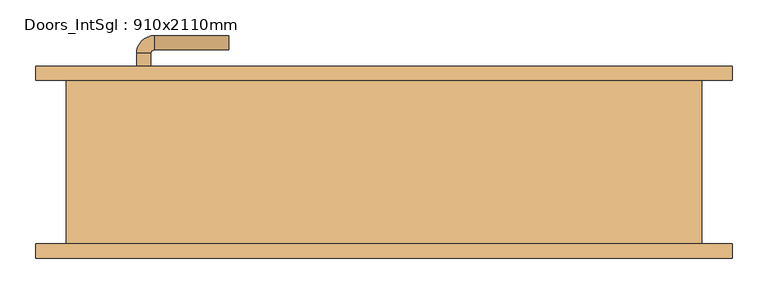
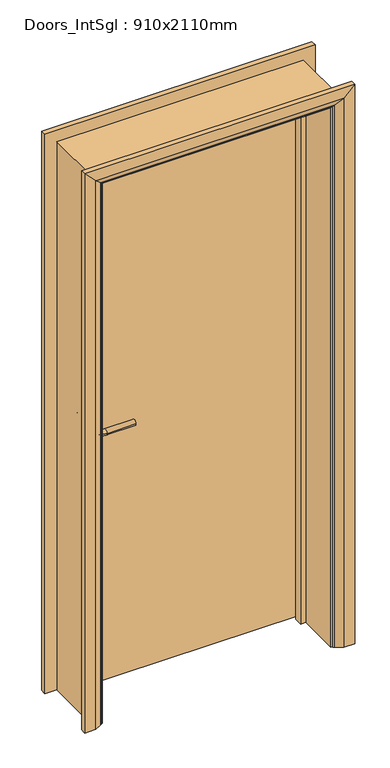
"""IFC4 building model written with IfcOpenShell, lengths in millimetres: door geometry, Doors_IntSgl : 910x2110mm."""

from ifc_helpers import new_model, si_unit, point, frame, frame_2d, origin, place, context, project, spatial, polyline, circle_curve, ellipse_curve, trimmed, segment, composite_curve, outline, extrude, faceted_brep, source, transform, mapped, element, save
from ifc_brep_helpers import plane_surface, cylinder_surface, revolved_surface, advanced_brep


def doors_intsgl_910x2110mm_0ed93a32(model_context):
    return source(origin(), model_context, "Body", "SolidModel", [
        advanced_brep(
        [(-348.0, 69.0, 1000.0), (-328.0, 69.0, 1000.0), (-328.0, 39.0, 1000.0), (-348.0, 39.0, 1000.0), (-323.0, 34.0, 1000.0), (-323.0, 14.0, 1000.0), (-218.0, 14.0, 1000.0), (-218.0, 34.0, 1000.0)],
        [
            (0, 1, circle_curve(frame((-338.0, 69.0, 1000.0), z_axis=(0.0, 1.0, 0.0), x_axis=(1.0, 0.0, 0.0)), 10.0)),
            (1, 0, circle_curve(frame((-338.0, 69.0, 1000.0), z_axis=(0.0, 1.0, 0.0), x_axis=(1.0, 0.0, 0.0)), 10.0)),
            (1, 2),
            (2, 3, circle_curve(frame((-338.0, 39.0, 1000.0), z_axis=(0.0, 1.0, 0.0), x_axis=(1.0, 0.0, 0.0)), 10.0)),
            (3, 0),
            (3, 2, circle_curve(frame((-338.0, 39.0, 1000.0), z_axis=(0.0, 1.0, 0.0), x_axis=(1.0, 0.0, 0.0)), 10.0)),
            (4, 5, circle_curve(frame((-323.0, 24.0, 1000.0), z_axis=(-1.0, 0.0, 0.0), x_axis=(0.0, 1.0, 0.0)), 10.0)),
            (5, 3, circle_curve(frame((-323.0, 39.0, 1000.0), z_axis=(0.0, 0.0, -1.0), x_axis=(-1.0, 0.0, 0.0)), 25.0)),
            (2, 4, circle_curve(frame((-323.0, 39.0, 1000.0), z_axis=(0.0, 0.0, 1.0), x_axis=(-1.0, 0.0, 0.0)), 5.0)),
            (5, 4, circle_curve(frame((-323.0, 24.0, 1000.0), z_axis=(-1.0, 0.0, 0.0), x_axis=(0.0, 1.0, 0.0)), 10.0)),
            (6, 7, circle_curve(frame((-218.0, 24.0, 1000.0), z_axis=(1.0, 0.0, 0.0), x_axis=(0.0, 1.0, 0.0)), 10.0)),
            (7, 6, circle_curve(frame((-218.0, 24.0, 1000.0), z_axis=(1.0, 0.0, 0.0), x_axis=(0.0, 1.0, 0.0)), 10.0)),
            (4, 7),
            (6, 5),
        ],
        [
            plane_surface(frame((-338.0, 69.0, 1000.0), z_axis=(0.0, 1.0, 0.0), x_axis=(0.0, 0.0, 1.0))),
            cylinder_surface(frame((-338.0, 69.0, 1000.0), z_axis=(0.0, 1.0, 0.0), x_axis=(1.0, 0.0, 0.0)), 10.0),
            revolved_surface(trimmed(ellipse_curve(frame((-338.0, 39.0, 1000.0), z_axis=(0.0, -1.0, 0.0), x_axis=(1.0, 0.0, 0.0)), 10.0, 10.0), [point((-348.0, 39.0, 1000.0))], [point((-328.0, 39.0, 1000.0))], True, "CARTESIAN"), (-323.0, 39.0, 1000.0), (0.0, 0.0, -1.0)),
            revolved_surface(trimmed(ellipse_curve(frame((-338.0, 39.0, 1000.0), z_axis=(0.0, -1.0, 0.0), x_axis=(1.0, 0.0, 0.0)), 10.0, 10.0), [point((-328.0, 39.0, 1000.0))], [point((-348.0, 39.0, 1000.0))], True, "CARTESIAN"), (-323.0, 39.0, 1000.0), (0.0, 0.0, -1.0)),
            plane_surface(frame((-218.0, 24.0, 1000.0), z_axis=(1.0, 0.0, 0.0), x_axis=(0.0, 0.0, 1.0))),
            cylinder_surface(frame((-323.0, 24.0, 1000.0), z_axis=(-1.0, 0.0, 0.0), x_axis=(0.0, 1.0, 0.0)), 10.0),
        ],
        [
            (0, [[1, 2]]),
            (1, [[3, 4, 5, -2]]),
            (1, [[-5, 6, -3, -1]]),
            (2, [[7, 8, -4, 9]]),
            (3, [[10, -9, -6, -8]]),
            (4, [[11, 12]]),
            (5, [[13, -11, 14, -7]]),
            (5, [[-14, -12, -13, -10]]),
        ],
    ),
        extrude(outline(composite_curve([segment(trimmed(circle_curve(frame_2d((1000.0, -340.5)), 30.0), [point((1000.0, -370.5))], [point((1000.0, -310.5))], False, "CARTESIAN"), True, "CONTINUOUS"), segment(trimmed(circle_curve(frame_2d((1000.0, -340.5)), 30.0), [point((1000.0, -310.5))], [point((1000.0, -370.5))], False, "CARTESIAN"), True, "CONTINUOUS")], self_intersect=False)), frame((0.0, 69.0, 0.0), z_axis=(0.0, 1.0, 0.0), x_axis=(0.0, 0.0, 1.0)), (0.0, 0.0, 1.0), 8.0),
        advanced_brep(
        [(-348.0, 123.0, 1000.0), (-328.0, 123.0, 1000.0), (-348.0, 153.0, 1000.0), (-328.0, 153.0, 1000.0), (-323.0, 158.0, 1000.0), (-323.0, 178.0, 1000.0), (-218.0, 178.0, 1000.0), (-218.0, 158.0, 1000.0)],
        [
            (0, 1, circle_curve(frame((-338.0, 123.0, 1000.0), z_axis=(0.0, -1.0, 0.0), x_axis=(1.0, 0.0, 0.0)), 10.0)),
            (1, 0, circle_curve(frame((-338.0, 123.0, 1000.0), z_axis=(0.0, -1.0, 0.0), x_axis=(1.0, 0.0, 0.0)), 10.0)),
            (0, 2),
            (2, 3, circle_curve(frame((-338.0, 153.0, 1000.0), z_axis=(0.0, -1.0, 0.0), x_axis=(1.0, 0.0, 0.0)), 10.0)),
            (3, 1),
            (3, 2, circle_curve(frame((-338.0, 153.0, 1000.0), z_axis=(0.0, -1.0, 0.0), x_axis=(1.0, 0.0, 0.0)), 10.0)),
            (4, 3, circle_curve(frame((-323.0, 153.0, 1000.0), z_axis=(0.0, 0.0, 1.0), x_axis=(-1.0, 0.0, 0.0)), 5.0)),
            (2, 5, circle_curve(frame((-323.0, 153.0, 1000.0), z_axis=(0.0, 0.0, -1.0), x_axis=(-1.0, 0.0, 0.0)), 25.0)),
            (5, 4, circle_curve(frame((-323.0, 168.0, 1000.0), z_axis=(-1.0, 0.0, 0.0), x_axis=(0.0, -1.0, 0.0)), 10.0)),
            (4, 5, circle_curve(frame((-323.0, 168.0, 1000.0), z_axis=(-1.0, 0.0, 0.0), x_axis=(0.0, -1.0, 0.0)), 10.0)),
            (6, 7, circle_curve(frame((-218.0, 168.0, 1000.0), z_axis=(1.0, 0.0, 0.0), x_axis=(0.0, -1.0, 0.0)), 10.0)),
            (7, 6, circle_curve(frame((-218.0, 168.0, 1000.0), z_axis=(1.0, 0.0, 0.0), x_axis=(0.0, -1.0, 0.0)), 10.0)),
            (5, 6),
            (7, 4),
        ],
        [
            plane_surface(frame((-338.0, 123.0, 1000.0), z_axis=(0.0, -1.0, 0.0), x_axis=(0.0, 0.0, 1.0))),
            cylinder_surface(frame((-338.0, 123.0, 1000.0), z_axis=(0.0, -1.0, 0.0), x_axis=(1.0, 0.0, 0.0)), 10.0),
            revolved_surface(trimmed(ellipse_curve(frame((-338.0, 153.0, 1000.0), z_axis=(0.0, -1.0, 0.0), x_axis=(1.0, 0.0, 0.0)), 10.0, 10.0), [point((-348.0, 153.0, 1000.0))], [point((-328.0, 153.0, 1000.0))], True, "CARTESIAN"), (-323.0, 153.0, 1000.0), (0.0, 0.0, -1.0)),
            revolved_surface(trimmed(ellipse_curve(frame((-338.0, 153.0, 1000.0), z_axis=(0.0, -1.0, 0.0), x_axis=(1.0, 0.0, 0.0)), 10.0, 10.0), [point((-328.0, 153.0, 1000.0))], [point((-348.0, 153.0, 1000.0))], True, "CARTESIAN"), (-323.0, 153.0, 1000.0), (0.0, 0.0, -1.0)),
            plane_surface(frame((-218.0, 168.0, 1000.0), z_axis=(1.0, 0.0, 0.0), x_axis=(0.0, 0.0, 1.0))),
            cylinder_surface(frame((-323.0, 168.0, 1000.0), z_axis=(-1.0, 0.0, 0.0), x_axis=(0.0, -1.0, 0.0)), 10.0),
        ],
        [
            (0, [[1, 2]]),
            (1, [[-1, 3, 4, 5]]),
            (1, [[-2, -5, 6, -3]]),
            (2, [[7, -4, 8, 9]]),
            (3, [[-8, -6, -7, 10]]),
            (4, [[11, 12]]),
            (5, [[-9, 13, -12, 14]]),
            (5, [[-10, -14, -11, -13]]),
        ],
    ),
        extrude(outline(composite_curve([segment(trimmed(circle_curve(frame_2d((1000.0, -340.5)), 30.0), [point((1000.0, -370.5))], [point((1000.0, -310.5))], False, "CARTESIAN"), True, "CONTINUOUS"), segment(trimmed(circle_curve(frame_2d((1000.0, -340.5)), 30.0), [point((1000.0, -310.5))], [point((1000.0, -370.5))], False, "CARTESIAN"), True, "CONTINUOUS")], self_intersect=False)), frame((0.0, 115.0, 0.0), z_axis=(0.0, 1.0, 0.0), x_axis=(0.0, 0.0, 1.0)), (0.0, 0.0, 1.0), 8.0),
        extrude(outline(polyline([(413.0, 77.0), (-413.0, 77.0), (-413.0, 115.0), (413.0, 115.0), (413.0, 77.0)])), frame((0.0, 0.0, 8.0), z_axis=(0.0, 0.0, 1.0), x_axis=(1.0, 0.0, 0.0)), (0.0, 0.0, 1.0), 2060.0),
        advanced_brep(
        [(490.0, 135.0, 0.0), (490.0, 115.0, 0.0), (420.0, 115.0, 0.0), (424.0, 121.0, 0.0), (450.0, 135.0, 0.0), (490.0, 135.0, 2145.0), (490.0, 115.0, 2145.0), (-490.0, 115.0, 2145.0), (-490.0, 115.0, 0.0), (-420.0, 115.0, 0.0), (-420.0, 115.0, 2075.0), (420.0, 115.0, 2075.0), (424.0, 121.0, 2079.0), (450.0, 135.0, 2105.0), (-450.0, 135.0, 2105.0), (-450.0, 135.0, 0.0), (-490.0, 135.0, 0.0), (-490.0, 135.0, 2145.0), (-424.0, 121.0, 2079.0), (-424.0, 121.0, 0.0)],
        [
            (0, 1),
            (1, 2),
            (2, 3, circle_curve(frame((428.0, 114.0, 0.0), z_axis=(0.0, 0.0, -1.0), x_axis=(1.0, 0.0, 0.0)), 8.0622577)),
            (3, 4),
            (4, 0),
            (0, 5),
            (5, 6),
            (6, 1),
            (6, 7),
            (7, 8),
            (8, 9),
            (9, 10),
            (10, 11),
            (11, 2),
            (11, 12, ellipse_curve(frame((428.0, 114.0, 2083.0), z_axis=(0.7071067811865475, 0.0, -0.7071067811865475), x_axis=(-0.7071067811865474, 0.0, -0.7071067811865476)), 11.4017543, 8.0622577)),
            (12, 3),
            (12, 13),
            (13, 4),
            (13, 14),
            (14, 15),
            (15, 16),
            (16, 17),
            (17, 5),
            (17, 7),
            (10, 18, ellipse_curve(frame((-428.0, 114.0, 2083.0), z_axis=(0.7071067811865475, 0.0, 0.7071067811865475), x_axis=(0.7071067811865476, 0.0, -0.7071067811865474)), 11.4017543, 8.0622577)),
            (18, 12),
            (18, 14),
            (15, 19),
            (19, 9, circle_curve(frame((-428.0, 114.0, 0.0), z_axis=(0.0, 0.0, -1.0), x_axis=(-1.0, 0.0, 0.0)), 8.0622577)),
            (8, 16),
            (19, 18),
        ],
        [
            plane_surface(frame((420.0, 115.0, 0.0), z_axis=(0.0, 0.0, -1.0), x_axis=(0.0, -1.0, 0.0))),
            plane_surface(frame((490.0, 135.0, 0.0), z_axis=(1.0, 0.0, 0.0), x_axis=(0.0, 0.0, 1.0))),
            plane_surface(frame((490.0, 115.0, 0.0), z_axis=(0.0, -1.0, 0.0), x_axis=(0.0, 0.0, 1.0))),
            cylinder_surface(frame((428.0, 114.0, 0.0), z_axis=(0.0, 0.0, -1.0), x_axis=(1.0, 0.0, 0.0)), 8.0622577),
            plane_surface(frame((424.0, 121.0, 0.0), z_axis=(-0.4740998230350126, 0.880471099922178, 0.0), x_axis=(0.0, 0.0, 1.0))),
            plane_surface(frame((450.0, 135.0, 0.0), z_axis=(0.0, 1.0, 0.0), x_axis=(0.0, 0.0, 1.0))),
            plane_surface(frame((490.0, 135.0, 2145.0), z_axis=(0.0, 0.0, 1.0), x_axis=(-1.0, 0.0, 0.0))),
            cylinder_surface(frame((420.0, 114.0, 2083.0), z_axis=(1.0, 0.0, 0.0), x_axis=(0.0, 0.0, 1.0)), 8.0622577),
            plane_surface(frame((424.0, 121.0, 2079.0), z_axis=(0.0, 0.8804710999221764, -0.4740998230350154), x_axis=(-1.0, 0.0, 0.0))),
            plane_surface(frame((-420.0, 115.0, 0.0), z_axis=(0.0, 0.0, -1.0), x_axis=(0.0, -1.0, 0.0))),
            plane_surface(frame((-490.0, 135.0, 2145.0), z_axis=(-1.0, 0.0, 0.0), x_axis=(0.0, 0.0, -1.0))),
            cylinder_surface(frame((-428.0, 114.0, 2075.0), z_axis=(0.0, 0.0, 1.0), x_axis=(-1.0, 0.0, 0.0)), 8.0622577),
            plane_surface(frame((-424.0, 121.0, 2079.0), z_axis=(0.47409982303501824, 0.8804710999221749, 0.0), x_axis=(0.0, 0.0, -1.0))),
        ],
        [
            (0, [[1, 2, 3, 4, 5]]),
            (1, [[-1, 6, 7, 8]]),
            (2, [[-2, -8, 9, 10, 11, 12, 13, 14]]),
            (3, [[-3, -14, 15, 16]]),
            (4, [[-4, -16, 17, 18]]),
            (5, [[-5, -18, 19, 20, 21, 22, 23, -6]]),
            (6, [[-7, -23, 24, -9]]),
            (7, [[-15, -13, 25, 26]]),
            (8, [[-17, -26, 27, -19]]),
            (9, [[-21, 28, 29, -11, 30]]),
            (10, [[-24, -22, -30, -10]]),
            (11, [[-25, -12, -29, 31]]),
            (12, [[-27, -31, -28, -20]]),
        ],
    ),
        extrude(outline(polyline([(0.0, -415.0), (0.0, -396.0), (2051.0, -396.0), (2051.0, 396.0), (0.0, 396.0), (0.0, 415.0), (2070.0, 415.0), (2070.0, -415.0), (0.0, -415.0)])), frame((0.0, 43.0, 0.0), z_axis=(0.0, 1.0, 0.0), x_axis=(0.0, 0.0, 1.0)), (0.0, 0.0, 1.0), 32.0),
        advanced_brep(
        [(-490.0, -135.0, 0.0), (-490.0, -115.0, 0.0), (-420.0, -115.0, 0.0), (-424.0, -121.0, 0.0), (-450.0, -135.0, 0.0), (-490.0, -135.0, 2145.0), (-490.0, -115.0, 2145.0), (-420.0, -115.0, 2075.0), (-424.0, -121.0, 2079.0), (-450.0, -135.0, 2105.0), (490.0, -135.0, 2145.0), (490.0, -115.0, 2145.0), (420.0, -115.0, 2075.0), (424.0, -121.0, 2079.0), (450.0, -135.0, 2105.0), (490.0, -135.0, 0.0), (450.0, -135.0, 0.0), (424.0, -121.0, 0.0), (420.0, -115.0, 0.0), (490.0, -115.0, 0.0)],
        [
            (0, 1),
            (1, 2),
            (2, 3, circle_curve(frame((-428.0, -114.0, 0.0), z_axis=(0.0, 0.0, -1.0), x_axis=(-1.0, 0.0, 0.0)), 8.0622577)),
            (3, 4),
            (4, 0),
            (0, 5),
            (5, 6),
            (6, 1),
            (6, 7),
            (7, 2),
            (7, 8, ellipse_curve(frame((-428.0, -114.0, 2083.0), z_axis=(-0.7071067811865475, 0.0, -0.7071067811865475), x_axis=(0.7071067811865474, 0.0, -0.7071067811865476)), 11.4017543, 8.0622577)),
            (8, 3),
            (8, 9),
            (9, 4),
            (9, 5),
            (5, 10),
            (10, 11),
            (11, 6),
            (11, 12),
            (12, 7),
            (12, 13, ellipse_curve(frame((428.0, -114.0, 2083.0), z_axis=(-0.7071067811865475, 0.0, 0.7071067811865475), x_axis=(-0.7071067811865476, 0.0, -0.7071067811865474)), 11.4017543, 8.0622577)),
            (13, 8),
            (13, 14),
            (14, 9),
            (14, 10),
            (15, 16),
            (16, 17),
            (17, 18, circle_curve(frame((428.0, -114.0, 0.0), z_axis=(0.0, 0.0, -1.0), x_axis=(1.0, 0.0, 0.0)), 8.0622577)),
            (18, 19),
            (19, 15),
            (10, 15),
            (19, 11),
            (18, 12),
            (17, 13),
            (16, 14),
        ],
        [
            plane_surface(frame((-420.0, -187.8010989, 0.0), z_axis=(0.0, 0.0, -1.0), x_axis=(1.0, 0.0, 0.0))),
            plane_surface(frame((-490.0, -135.0, 0.0), z_axis=(-1.0, 0.0, 0.0), x_axis=(0.0, 0.0, 1.0))),
            plane_surface(frame((-490.0, -115.0, 0.0), z_axis=(0.0, 1.0, 0.0), x_axis=(0.0, 0.0, 1.0))),
            cylinder_surface(frame((-428.0, -114.0, 0.0), z_axis=(0.0, 0.0, -1.0), x_axis=(-1.0, 0.0, 0.0)), 8.0622577),
            plane_surface(frame((-424.0, -121.0, 0.0), z_axis=(0.4740998230350183, -0.8804710999221749, 0.0), x_axis=(0.0, 0.0, 1.0))),
            plane_surface(frame((-450.0, -135.0, 0.0), z_axis=(0.0, -1.0, 0.0), x_axis=(0.0, 0.0, 1.0))),
            plane_surface(frame((-490.0, -135.0, 2145.0), z_axis=(0.0, 0.0, 1.0), x_axis=(1.0, 0.0, 0.0))),
            plane_surface(frame((-490.0, -115.0, 2145.0), z_axis=(0.0, 1.0, 0.0), x_axis=(1.0, 0.0, 0.0))),
            cylinder_surface(frame((-420.0, -114.0, 2083.0), z_axis=(-1.0, 0.0, 0.0), x_axis=(0.0, 0.0, 1.0)), 8.0622577),
            plane_surface(frame((-424.0, -121.0, 2079.0), z_axis=(0.0, -0.8804710999221749, -0.4740998230350183), x_axis=(1.0, 0.0, 0.0))),
            plane_surface(frame((-450.0, -135.0, 2105.0), z_axis=(0.0, -1.0, 0.0), x_axis=(1.0, 0.0, 0.0))),
            plane_surface(frame((420.0, -187.8010989, 0.0), z_axis=(0.0, 0.0, -1.0), x_axis=(-1.0, 0.0, 0.0))),
            plane_surface(frame((490.0, -135.0, 2145.0), z_axis=(1.0, 0.0, 0.0), x_axis=(0.0, 0.0, -1.0))),
            plane_surface(frame((490.0, -115.0, 2145.0), z_axis=(0.0, 1.0, 0.0), x_axis=(0.0, 0.0, -1.0))),
            cylinder_surface(frame((428.0, -114.0, 2075.0), z_axis=(0.0, 0.0, 1.0), x_axis=(1.0, 0.0, 0.0)), 8.0622577),
            plane_surface(frame((424.0, -121.0, 2079.0), z_axis=(-0.4740998230350183, -0.8804710999221749, 0.0), x_axis=(0.0, 0.0, -1.0))),
            plane_surface(frame((450.0, -135.0, 2105.0), z_axis=(0.0, -1.0, 0.0), x_axis=(0.0, 0.0, -1.0))),
        ],
        [
            (0, [[1, 2, 3, 4, 5]]),
            (1, [[-1, 6, 7, 8]]),
            (2, [[-2, -8, 9, 10]]),
            (3, [[-3, -10, 11, 12]]),
            (4, [[-4, -12, 13, 14]]),
            (5, [[-5, -14, 15, -6]]),
            (6, [[-7, 16, 17, 18]]),
            (7, [[-9, -18, 19, 20]]),
            (8, [[-11, -20, 21, 22]]),
            (9, [[-13, -22, 23, 24]]),
            (10, [[-15, -24, 25, -16]]),
            (11, [[26, 27, 28, 29, 30]]),
            (12, [[-17, 31, -30, 32]]),
            (13, [[-19, -32, -29, 33]]),
            (14, [[-21, -33, -28, 34]]),
            (15, [[-23, -34, -27, 35]]),
            (16, [[-25, -35, -26, -31]]),
        ],
    ),
        faceted_brep([(-415.0, 115.0, 0.0), (-415.0, -115.0, 0.0), (-447.0, -115.0, 0.0), (-447.0, 115.0, 0.0), (-415.0, 115.0, 2070.0), (-415.0, -115.0, 2070.0), (-447.0, -115.0, 2102.0), (-447.0, 115.0, 2102.0), (415.0, 115.0, 2070.0), (415.0, -115.0, 2070.0), (447.0, -115.0, 2102.0), (447.0, 115.0, 2102.0), (415.0, 115.0, 0.0), (447.0, 115.0, 0.0), (447.0, -115.0, 0.0), (415.0, -115.0, 0.0)], [[[0, 1, 2, 3]], [[1, 0, 4, 5]], [[2, 1, 5, 6]], [[3, 2, 6, 7]], [[0, 3, 7, 4]], [[5, 4, 8, 9]], [[6, 5, 9, 10]], [[7, 6, 10, 11]], [[4, 7, 11, 8]], [[12, 13, 14, 15]], [[9, 8, 12, 15]], [[10, 9, 15, 14]], [[11, 10, 14, 13]], [[8, 11, 13, 12]]]),
    ])


if __name__ == "__main__":
    model = new_model("IFC4")
    model_context = context("Model", 3, world=origin())
    ifc_project = project(units=[si_unit("LENGTHUNIT", "METRE", prefix="MILLI")], contexts=[model_context])
    site = spatial("IfcSite", under=ifc_project)
    building = spatial("IfcBuilding", under=site)
    placement = place(None, origin())
    doors_intsgl_910x2110mm_shape = doors_intsgl_910x2110mm_0ed93a32(model_context)
    element("IfcDoor", 1, ObjectType="Doors_IntSgl : 910x2110mm", at=placement, inside=building, context=model_context, shape_type="MappedRepresentation", body=[
        mapped(doors_intsgl_910x2110mm_shape, transform((0.0, 0.0, 0.0), x_axis=(1.0, 0.0, 0.0), y_axis=(0.0, 1.0, 0.0), z_axis=(0.0, 0.0, 1.0))),
    ])
    save(model, "model.ifc")

# Revit data of these elements
# Type "Doors_IntSgl : 910x2110mm"
#   Construction Type Id = "MDOOR"
#   Type Mark = "41"
#   Type Comments = "Internal Single"
#   Operation = "SingleSwingRight"
#   Manufacturer = "Revit"
#   Keynote = "L20"
#   Description = "Internal Single Door"
#   Analytic Construction = "Metal"
#   UnderCut = 8 mm
#   Tolerance = 2 mm
#   Thickness = 38 mm
#   Thermal Resistance (R) = 0.270117 (m²·K)/W
#   Structural Tolerance = 8 mm
#   StopDepth = 32 mm
#   Stop Thickness = 19 mm
#   Rough Width = 910 mm
#   Rough Height = 2110 mm
#   Height to Top Lock Rail = 1000 mm
#   Heat Transfer Coefficient (U) = 3.7021 W/(m²·K)
#   Handle Z Distance = 1000 mm
#   Handle X Distance = 75 mm
#   Frame Thickness = 32 mm
#   Door Panel Width = 826 mm
#   Door Panel Thickness = 38 mm
#   Door Panel Offset = 0 mm
#   Height = 2110 mm
#   Width = 910 mm
#   Door Panel Height = 2060 mm
#   Architrave Setback = 5 mm
#   Define Thermal Properties by = 1
#   Vis - Ironmongery = yes
#   Material Ironmongery = Door - Handle
#   Material Frame = Door - Frame/Mullion (1)
#   Material Door = Door - Panel
#   Material Architrave = Door - Architrave
#   Visual Light Transmittance = 0
#   Solar Heat Gain Coefficient = 0
#   Function = (empty or 0)
#   Wall Closure = (empty or 0)
# Element 1 (IfcDoor, "Doors_IntSgl : 910x2110mm")
#   Materials on its faces: "Door - Architrave", "Door - Handle", "Door - Frame/Mullion (1)", "Door - Panel"
# Materials
#   "Door - Handle": class "Miscellaneous", colour RGB 0 0 0, transparency 0, Keynote = "P21", Cost = 0
#   "Door - Frame/Mullion (1)": class "Wood", colour RGB 212 179 113, transparency 0, Keynote = "L20", Cost = 0
#   "Door - Panel": class "Wood", colour RGB 210 159 95, transparency 0, Keynote = "L20", Cost = 0
#   "Door - Architrave": class "Wood", colour RGB 154 90 5, transparency 0, Keynote = "P20", Cost = 0
